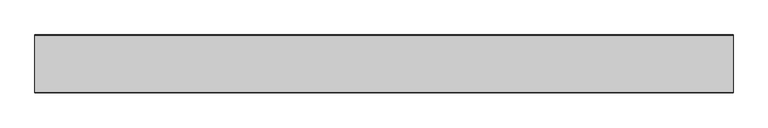
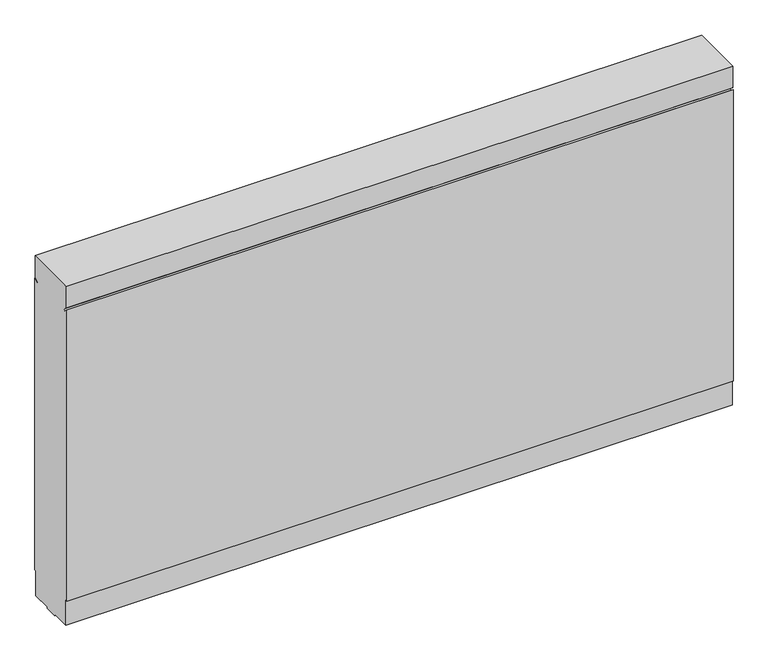
"""IFC4 building model written with IfcOpenShell, lengths in millimetres: proxy geometry, Generic Models 7:Generic Models 1:5:Generic Models 1:5 : Generic Models 7:Generic Models 1:337419:15 : Generic Models 7:Generic Models 1:5:Generic Models 1:5 : Generic Models 7:Generic Models 1:337419:311462."""

from ifc_helpers import new_model, si_unit, frame, origin, place, context, project, spatial, polyline, outline, extrude, source, transform, mapped, element, save


def generic_models_246ae870(model_context):
    return source(origin(), model_context, "Body", "SweptSolid", [
        extrude(outline(polyline([(-578799.0788841, 103.1875), (-578805.4288841, 103.1875), (-578805.4288841, 7.9375), (-578875.2788841, 7.9375), (-578875.2788841, 1.5875), (-578922.9038841, 1.5875), (-578922.9038841, 7.9375), (-578992.7538841, 7.9375), (-578992.7538841, 103.1875), (-578999.1038841, 103.1875), (-578999.1038841, 1217.1846578), (-578985.9025672, 1206.1074377), (-578982.0759722, 1210.667796), (-578996.3257591, 1222.6247869), (-578996.3257591, 1304.8288409), (-578801.8570091, 1304.8288409), (-578801.8570091, 1222.6247869), (-578816.1067959, 1210.667796), (-578812.2802009, 1206.1074376), (-578799.0788841, 1217.1846577), (-578799.0788841, 103.1875)])), frame((570490.7367239, 0.0, 0.0), z_axis=(1.0, 0.0, 0.0), x_axis=(0.0, 1.0, 0.0)), (0.0, 0.0, 1.0), 2406.65),
    ])


if __name__ == "__main__":
    model = new_model("IFC4")
    model_context = context("Model", 3, world=origin())
    ifc_project = project(units=[si_unit("LENGTHUNIT", "METRE", prefix="MILLI")], contexts=[model_context])
    site = spatial("IfcSite", under=ifc_project)
    building = spatial("IfcBuilding", under=site)
    placement = place(None, origin())
    generic_models_shape = generic_models_246ae870(model_context)
    element("IfcBuildingElementProxy", 1, Name="Generic Models 7:Generic Models 1:5:Generic Models 1:5 : Generic Models 7:Generic Models 1:337419:15 : Generic Models 7:Generic Models 1:5:Generic Models 1:5 : Generic Models 7:Generic Models 1:337419:311462", ObjectType="Generic Models 7:Generic Models 1:5:Generic Models 1:5 : Generic Models 7:Generic Models 1:337419:15 : Generic Models 7:Generic Models 1:5:Generic Models 1:5 : Generic Models 7:Generic Models 1:337419:311462", at=placement, inside=building, context=model_context, shape_type="MappedRepresentation", body=[
        mapped(generic_models_shape, transform((0.0, 0.0, 0.0), x_axis=(1.0, 0.0, 0.0), y_axis=(0.0, 1.0, 0.0), z_axis=(0.0, 0.0, 1.0))),
    ])
    save(model, "model.ifc")

# Revit data of these elements
# Type "Generic Models 7:Generic Models 1:5:Generic Models 1:5 : Generic Models 7:Generic Models 1:337419:15 : Generic Models 7:Generic Models 1:5:Generic Models 1:5 : Generic Models 7:Generic Models 1:337419:311462"
#   NameOverride = "Generic Models 7:Generic Models 1:5:Generic Models 1:5 : Generic Models 7:Generic Models 1:337419:311462"
#   ObjectTypeOverride = "Generic Models 1:5 : Generic Models 7:Generic Models 1:337419"
#   Reference = "Generic Models 1"
#   Tag = "311462"
